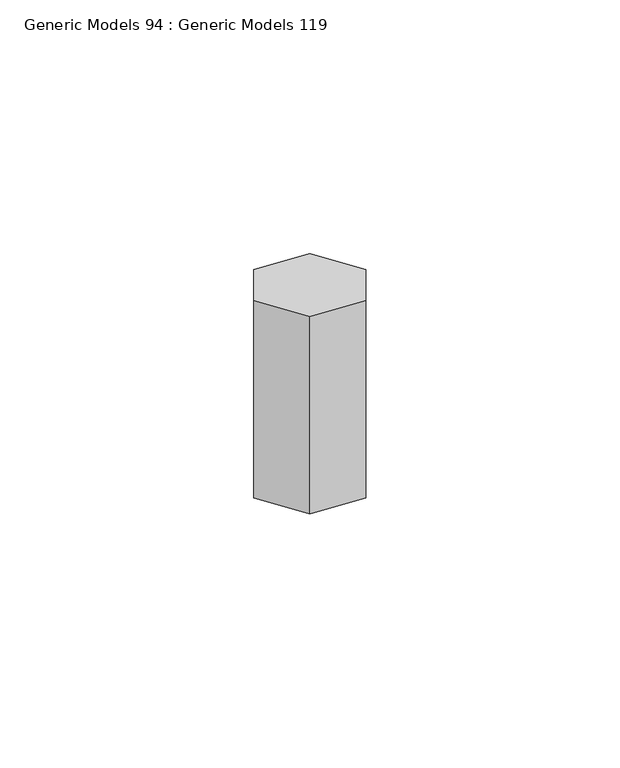
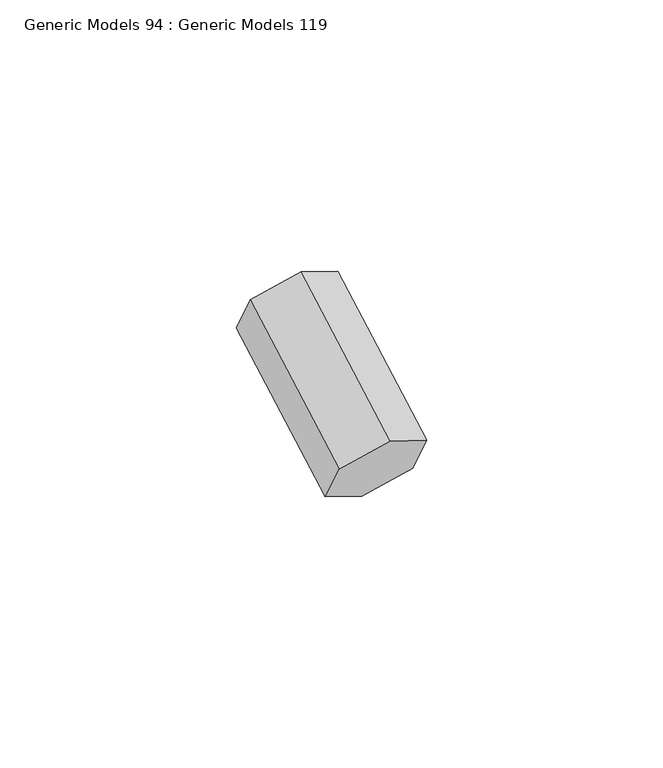
"""IFC4 building model written with IfcOpenShell, lengths in millimetres: proxy geometry, Generic Models 94 : Generic Models 119."""

from ifc_helpers import new_model, si_unit, frame, origin, place, context, project, spatial, polyline, outline, extrude, source, transform, mapped, element, save


def generic_models_94_generic_models_119_84900088(model_context):
    return source(origin(), model_context, "Body", "SweptSolid", [
        extrude(outline(polyline([(-6.3500001, 10.9985226), (6.35, 10.9985226), (12.6999999, 0.0), (6.35, -10.9985226), (-6.3500001, -10.9985226), (-12.7, 0.0), (-6.3500001, 10.9985226)])), frame((32003.9965778, 35133.6205521, 271581.1589661), z_axis=(0.0, 0.874619707139422, 0.4848096202462898), x_axis=(0.0, 0.4848096202462898, -0.874619707139422)), (0.0, 0.0, 1.0), 44.45),
    ])


if __name__ == "__main__":
    model = new_model("IFC4")
    model_context = context("Model", 3, world=origin())
    ifc_project = project(units=[si_unit("LENGTHUNIT", "METRE", prefix="MILLI")], contexts=[model_context])
    site = spatial("IfcSite", under=ifc_project)
    building = spatial("IfcBuilding", under=site)
    placement = place(None, origin())
    generic_models_94_generic_models_119_shape = generic_models_94_generic_models_119_84900088(model_context)
    element("IfcBuildingElementProxy", 1, Name="Generic Models 94 : Generic Models 119", ObjectType="Generic Models 94 : Generic Models 119", at=placement, inside=building, context=model_context, shape_type="MappedRepresentation", body=[
        mapped(generic_models_94_generic_models_119_shape, transform((0.0, 0.0, 0.0), x_axis=(1.0, 0.0, 0.0), y_axis=(0.0, 1.0, 0.0), z_axis=(0.0, 0.0, 1.0))),
    ])
    save(model, "model.ifc")
